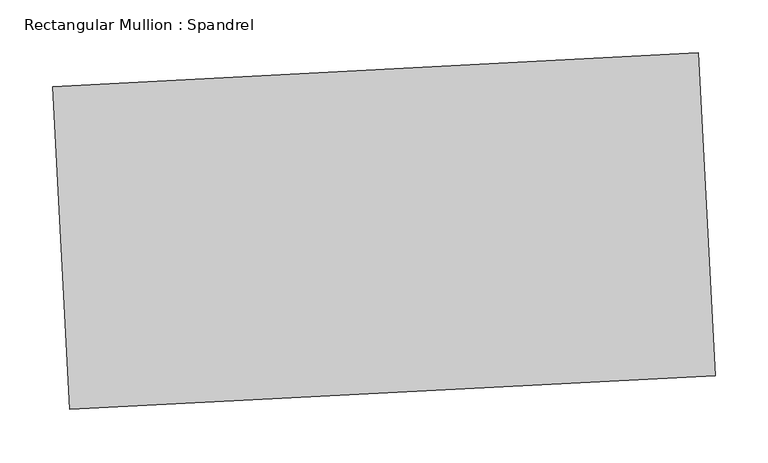
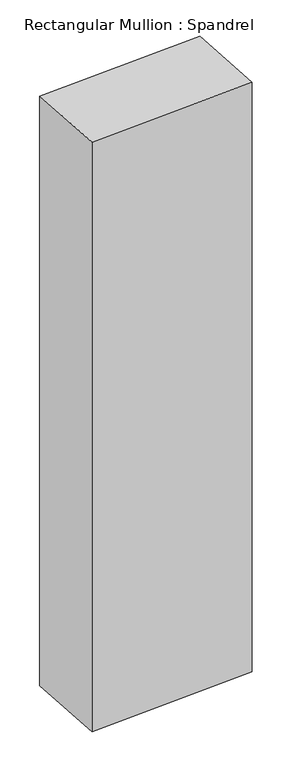
"""IFC4 building model written with IfcOpenShell, lengths in millimetres: member geometry, Rectangular Mullion : Spandrel."""

import ifcopenshell
import ifcopenshell.guid

model = None  # the IFC model being written
_history = None  # IfcOwnerHistory: only IFC2X3 demands one
_inside = {}  # id of a spatial element -> (the spatial element, [elements in it])
_under = {}  # id of a project, library or spatial element -> (it, [spatial elements below it])
_declared = {}  # id of a project -> (the project, [libraries it declares])
_typed = {}  # id of a type object -> (the type object, [elements of that type])
_made_of = {}  # id of a material, layer set ... -> (it, [elements and type objects made of it])


def new_model(schema):
    """Start an empty IFC model of exactly this schema.

    Asked for "IFC4X3", IfcOpenShell would pick the latest addendum, in which some entities
    have other attributes; the version numbers below select the first issue.
    IFC2X3 requires an IfcOwnerHistory on every rooted entity: one is made here for all.
    """
    global model, _history
    if schema == "IFC4X3":
        model = ifcopenshell.file(schema_version=(4, 3, 0, 0))
    else:
        model = ifcopenshell.file(schema=schema)
    _inside.clear()
    _under.clear()
    _declared.clear()
    _typed.clear()
    _made_of.clear()
    _history = None
    if model.schema == "IFC2X3":
        org = make("IfcOrganization", Name="unknown")
        user = make(
            "IfcPersonAndOrganization",
            ThePerson=make("IfcPerson", FamilyName="unknown"),
            TheOrganization=org,
        )
        app = make(
            "IfcApplication",
            ApplicationDeveloper=org,
            Version="unknown",
            ApplicationFullName="unknown",
            ApplicationIdentifier="unknown",
        )
        _history = make(
            "IfcOwnerHistory",
            OwningUser=user,
            OwningApplication=app,
            ChangeAction="ADDED",
            CreationDate=0,
        )
    return model


def make(cls, **values):
    """One entity of the class cls with the attributes given. An attribute that is None is left unset."""
    return model.create_entity(
        cls, **{name: value for name, value in values.items() if value is not None}
    )


def rooted(cls, **values):
    """An entity with a GlobalId (a new one), such as an element, a storey or a relation."""
    return make(cls, GlobalId=ifcopenshell.guid.new(), OwnerHistory=_history, **values)


def si_unit(unit_type, name, prefix=None):
    """IfcSIUnit, for example si_unit("LENGTHUNIT", "METRE", prefix="MILLI")."""
    return make("IfcSIUnit", UnitType=unit_type, Prefix=prefix, Name=name)


def assignment(units):
    """IfcUnitAssignment: the units of a project."""
    return None if units is None else make("IfcUnitAssignment", Units=units)


def point(xyz):
    """IfcCartesianPoint."""
    return None if xyz is None else make("IfcCartesianPoint", Coordinates=xyz)


def direction(xyz):
    """IfcDirection."""
    return None if xyz is None else make("IfcDirection", DirectionRatios=xyz)


def frame(location, z_axis=None, x_axis=None):
    """IfcAxis2Placement3D, a coordinate frame: its origin and axes. An axis left out is left unset."""
    return make(
        "IfcAxis2Placement3D",
        Location=point(location),
        Axis=direction(z_axis),
        RefDirection=direction(x_axis),
    )


def origin():
    """The frame at (0, 0, 0) with its axes left unset."""
    return frame((0.0, 0.0, 0.0))


def place(relative_to, where):
    """IfcLocalPlacement: puts the frame where relative to a parent placement (None: the world)."""
    return make(
        "IfcLocalPlacement", PlacementRelTo=relative_to, RelativePlacement=where
    )


def context(
    kind, dimensions, precision=None, world=None, true_north=None, identifier=None
):
    """IfcGeometricRepresentationContext, for example the 3D "Model" context."""
    return make(
        "IfcGeometricRepresentationContext",
        ContextIdentifier=identifier,
        ContextType=kind,
        CoordinateSpaceDimension=dimensions,
        Precision=precision,
        WorldCoordinateSystem=world,
        TrueNorth=true_north,
    )


def project(units=None, contexts=None):
    """IfcProject with its units and contexts."""
    return rooted(
        "IfcProject",
        Name="project",
        RepresentationContexts=contexts,
        UnitsInContext=assignment(units),
    )


def spatial(cls, under=None, at=None, **own):
    """A site, building, storey or space (cls), placed at a placement, below another one or the project."""
    s = rooted(cls, ObjectPlacement=at, **own)
    if under is not None:
        _under.setdefault(under.id(), (under, []))[1].append(s)
    return s


def polyline(points):
    """IfcPolyline through the points."""
    return make("IfcPolyline", Points=[point(p) for p in points])


def outline(outer, holes=None, kind="AREA"):
    """IfcArbitraryClosedProfileDef: a profile drawn as a closed curve; with holes, ...WithVoids."""
    if holes is None:
        return make("IfcArbitraryClosedProfileDef", ProfileType=kind, OuterCurve=outer)
    return make(
        "IfcArbitraryProfileDefWithVoids",
        ProfileType=kind,
        OuterCurve=outer,
        InnerCurves=holes,
    )


def extrude(swept, where, along, depth):
    """IfcExtrudedAreaSolid: the profile swept, set in the frame where, extruded along a direction by depth."""
    return make(
        "IfcExtrudedAreaSolid",
        SweptArea=swept,
        Position=where,
        ExtrudedDirection=direction(along),
        Depth=depth,
    )


def shape(context_of_items, identifier, shape_type, items):
    """IfcShapeRepresentation: the items that make up one representation, for example the "Body"."""
    return make(
        "IfcShapeRepresentation",
        ContextOfItems=context_of_items,
        RepresentationIdentifier=identifier,
        RepresentationType=shape_type,
        Items=items,
    )


def source(mapping_origin, context_of_items, identifier, shape_type, items):
    """IfcRepresentationMap: a shape defined once, which mapped items show again and again."""
    return make(
        "IfcRepresentationMap",
        MappingOrigin=mapping_origin,
        MappedRepresentation=shape(context_of_items, identifier, shape_type, items),
    )


def transform(
    local_origin,
    x_axis=None,
    y_axis=None,
    z_axis=None,
    scale=None,
    scale2=None,
    scale3=None,
    uniform=True,
):
    """IfcCartesianTransformationOperator3D, or its non-uniform kind. x_axis, y_axis, z_axis: its Axis1, 2, 3."""
    if uniform:
        return make(
            "IfcCartesianTransformationOperator3D",
            Axis1=direction(x_axis),
            Axis2=direction(y_axis),
            LocalOrigin=point(local_origin),
            Scale=scale,
            Axis3=direction(z_axis),
        )
    return make(
        "IfcCartesianTransformationOperator3DnonUniform",
        Axis1=direction(x_axis),
        Axis2=direction(y_axis),
        LocalOrigin=point(local_origin),
        Scale=scale,
        Axis3=direction(z_axis),
        Scale2=scale2,
        Scale3=scale3,
    )


def mapped(mapping_source, mapping_target):
    """IfcMappedItem: shows the shape of a source again, moved by a transform."""
    return make(
        "IfcMappedItem", MappingSource=mapping_source, MappingTarget=mapping_target
    )


def made_of(thing, what):
    """Note that an element or type object is made of a material, layer set ...; save() writes the relation."""
    if what is not None:
        _made_of.setdefault(what.id(), (what, []))[1].append(thing)
    return thing


def element(
    cls,
    number,
    at=None,
    inside=None,
    cuts=None,
    type_object=None,
    material=None,
    context=None,
    identifier="Body",
    shape_type=None,
    held_by="IfcProductDefinitionShape",
    body=None,
    shapes=None,
    **own,
):
    """One element of the class cls, such as IfcWall. Its Tag is "e" and its number.

    at: its placement. inside: the storey or other place that contains it. cuts: it is an
    opening in that element (IfcRelVoidsElement). A single representation is given by context,
    identifier, shape_type and body (its items); several are given by shapes. held_by: the class
    of the entity that holds the representations. save() writes the other relations.
    """
    e = rooted(cls, Tag="e%d" % number, ObjectPlacement=at, **own)
    if body is not None:
        shapes = [shape(context, identifier, shape_type, body)]
    if shapes is not None:
        e.Representation = make(held_by, Representations=shapes)
    if inside is not None:
        _inside.setdefault(inside.id(), (inside, []))[1].append(e)
    if cuts is not None:
        rooted(
            "IfcRelVoidsElement", RelatingBuildingElement=cuts, RelatedOpeningElement=e
        )
    if type_object is not None:
        _typed.setdefault(type_object.id(), (type_object, []))[1].append(e)
    return made_of(e, material)


def aggregate(whole, parts):
    """IfcRelAggregates: a whole, such as a stair, and the parts it consists of."""
    return rooted("IfcRelAggregates", RelatingObject=whole, RelatedObjects=parts)


def save(model, path):
    """Write the relations noted so far, then the file.

    IfcRelAggregates (storeys below a building ...), IfcRelContainedInSpatialStructure (elements
    in a storey), IfcRelDefinesByType, IfcRelAssociatesMaterial and IfcRelDeclares: one each for
    every whole, place, type object, material and project.
    """
    for whole, parts in _under.values():
        aggregate(whole, parts)
    for where, things in _inside.values():
        rooted(
            "IfcRelContainedInSpatialStructure",
            RelatedElements=things,
            RelatingStructure=where,
        )
    for kind, things in _typed.values():
        rooted("IfcRelDefinesByType", RelatedObjects=things, RelatingType=kind)
    for what, things in _made_of.values():
        rooted("IfcRelAssociatesMaterial", RelatedObjects=things, RelatingMaterial=what)
    for by, libraries in _declared.values():
        rooted("IfcRelDeclares", RelatingContext=by, RelatedDefinitions=libraries)
    model.write(path)


def rectangular_mullion_spandrel_c07370e7(model_context):
    return source(origin(), model_context, "Body", "SweptSolid", [
        extrude(outline(polyline([(-617.1582819, 136.2391416), (-8.3937175, 168.1431406), (7.5582819, -136.2391416), (-601.2062825, -168.1431406), (-617.1582819, 136.2391416)])), frame((0.0, 0.0, -2293.6958315), z_axis=(0.0, 0.0, 1.0), x_axis=(1.0, 0.0, 0.0)), (0.0, 0.0, 1.0), 2293.6958315),
    ])


if __name__ == "__main__":
    model = new_model("IFC4")
    model_context = context("Model", 3, world=origin())
    ifc_project = project(units=[si_unit("LENGTHUNIT", "METRE", prefix="MILLI")], contexts=[model_context])
    site = spatial("IfcSite", under=ifc_project)
    building = spatial("IfcBuilding", under=site)
    placement = place(None, origin())
    rectangular_mullion_spandrel_shape = rectangular_mullion_spandrel_c07370e7(model_context)
    element("IfcMember", 1, ObjectType="Rectangular Mullion : Spandrel", at=placement, inside=building, context=model_context, shape_type="MappedRepresentation", body=[
        mapped(rectangular_mullion_spandrel_shape, transform((0.0, 0.0, 0.0), x_axis=(1.0, 0.0, 0.0), y_axis=(0.0, 1.0, 0.0), z_axis=(0.0, 0.0, 1.0))),
    ])
    save(model, "model.ifc")

# Revit data of these elements
# Type "Rectangular Mullion : Spandrel"
#   built-in parameter 1007304 = 1 (stored number, unit not read)
#   built-in parameter 1007301 = 1 (stored number, unit not read)
#   built-in parameter 1007300 = 1 (stored number, unit not read)
# Element 1 (IfcMember, "Rectangular Mullion : Spandrel")
#   Materials on its faces: "Aluminum"
# Materials
#   "Aluminum": class "Metal", colour RGB 247 247 247, transparency 0, Description = "Aluminum 6061", Cost = 0
